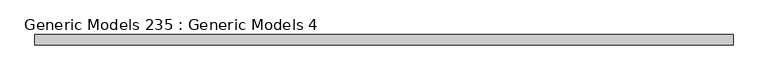
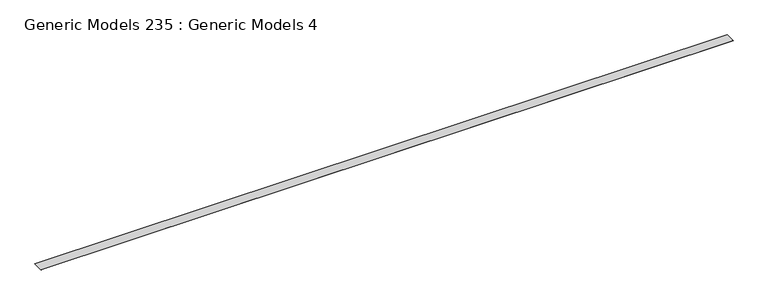
"""IFC4 building model written with IfcOpenShell, lengths in millimetres: proxy geometry, Generic Models 235 : Generic Models 4."""

from ifc_helpers import new_model, si_unit, frame, origin, place, context, project, spatial, polyline, outline, extrude, source, transform, mapped, element, save


def generic_models_235_generic_models_4_2af9478d(model_context):
    return source(origin(), model_context, "Body", "SweptSolid", [
        extrude(outline(polyline([(11503.7126626, 126939.6972134), (11784.3492027, 126939.6972134), (11784.3492344, 126938.9034634), (11503.7126626, 126938.8922805), (11503.7126626, 126939.6972134)])), frame((-10234.5171316, 0.0, 0.0), z_axis=(1.0, 0.0, 0.0), x_axis=(0.0, 1.0, 0.0)), (0.0, 0.0, 1.0), 18643.6),
    ])


if __name__ == "__main__":
    model = new_model("IFC4")
    model_context = context("Model", 3, world=origin())
    ifc_project = project(units=[si_unit("LENGTHUNIT", "METRE", prefix="MILLI")], contexts=[model_context])
    site = spatial("IfcSite", under=ifc_project)
    building = spatial("IfcBuilding", under=site)
    placement = place(None, origin())
    generic_models_235_generic_models_4_shape = generic_models_235_generic_models_4_2af9478d(model_context)
    element("IfcBuildingElementProxy", 1, Name="Generic Models 235 : Generic Models 4", ObjectType="Generic Models 235 : Generic Models 4", at=placement, inside=building, context=model_context, shape_type="MappedRepresentation", body=[
        mapped(generic_models_235_generic_models_4_shape, transform((0.0, 0.0, 0.0), x_axis=(1.0, 0.0, 0.0), y_axis=(0.0, 1.0, 0.0), z_axis=(0.0, 0.0, 1.0))),
    ])
    save(model, "model.ifc")

# Revit data of these elements
# Element 1 (IfcBuildingElementProxy, "Generic Models 235 : Generic Models 4")
#   Materials on its faces: "_HYDROSTOP LIQUID MEMBRANE - FOLLOW MANU. RECOMMENDED INSTALLATION DETAILS"
# Materials
#   "_HYDROSTOP LIQUID MEMBRANE - FOLLOW MANU. RECOMMENDED INSTALLATION DETAILS": class "Generic", colour RGB 156 184 169, transparency 0, Cost = 0
